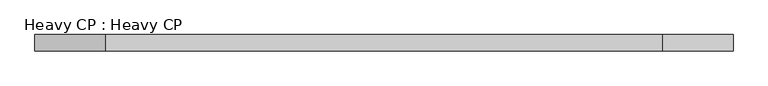
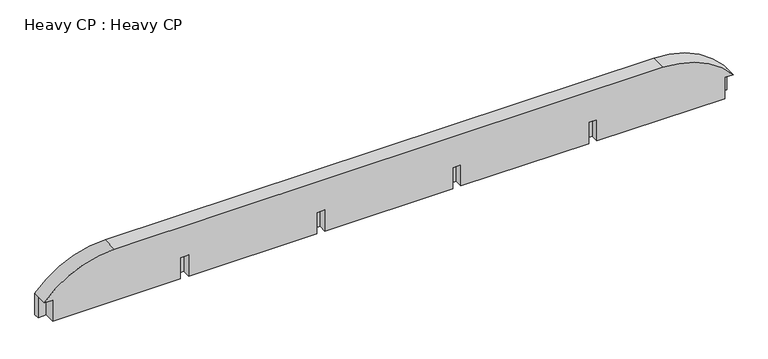
"""IFC4 building model written with IfcOpenShell, lengths in millimetres: beam geometry, Heavy CP : Heavy CP."""

from ifc_helpers import new_model, si_unit, frame, origin, place, context, project, spatial, circle_curve, source, transform, mapped, element, save
from ifc_brep_helpers import plane_surface, cylinder_surface, advanced_brep


def heavy_cp_heavy_cp_8a3f1562(model_context):
    return source(origin(), model_context, "Body", "AdvancedBrep", [
        advanced_brep(
        [(25183.2245516, 20299.9999993, 13800.0), (25183.2245516, 20299.9999993, 14620.0), (27758.2245515, 20299.9999993, 15800.827786), (47908.2245512, 20299.9999993, 15800.827786), (50483.2245514, 20299.9999993, 14619.9999997), (50483.2245514, 20299.9999993, 13800.0), (27583.2245516, 20299.9999993, 13800.0), (50483.2245514, 19699.9999993, 14619.9999997), (47908.2245512, 19699.9999993, 15800.827786), (27758.2245515, 19699.9999993, 15800.827786), (25183.2245516, 19699.9999993, 14620.0), (25483.2245516, 19699.9999993, 14620.0), (25483.2245516, 19699.9999993, 13800.0), (27583.2245516, 19699.9999993, 13800.0), (30183.2245515, 19699.9999993, 13800.0), (30183.2245515, 19699.9999993, 14620.0), (30333.2245515, 19699.9999993, 14620.0), (30483.2245515, 19699.9999993, 14620.0), (30483.2245515, 19699.9999993, 13800.0), (35183.2245514, 19699.9999993, 13800.0), (35183.2245514, 19699.9999993, 14620.0), (35483.2245514, 19699.9999993, 14620.0), (35483.2245514, 19699.9999993, 13800.0), (40183.2245513, 19699.9999993, 13800.0), (40183.2245513, 19699.9999993, 14620.0), (40483.2245513, 19699.9999993, 14620.0), (40483.2245513, 19699.9999993, 13800.0), (45183.2245512, 19699.9999993, 13800.0), (45183.2245512, 19699.9999993, 14620.0), (45483.2245512, 19699.9999993, 14620.0), (45483.2245512, 19699.9999993, 13800.0), (50183.2245511, 19699.9999993, 13800.0), (50183.2245511, 19699.9999993, 14620.0), (25183.2245516, 20099.7448193, 13800.0), (25183.2245516, 20099.7448193, 14620.0), (50483.2245511, 20099.7448193, 14620.0), (50483.2245514, 20099.7448193, 13800.0), (50183.2245511, 20099.7448193, 13800.0), (45483.2245512, 19999.9999993, 13800.0), (45183.2245512, 19999.9999993, 13800.0), (40483.2245513, 19999.9999993, 13800.0), (40183.2245513, 19999.9999993, 13800.0), (35483.2245514, 19999.9999993, 13800.0), (35183.2245514, 19999.9999993, 13800.0), (30483.2245515, 19999.9999993, 13800.0), (30183.2245515, 19999.9999993, 13800.0), (25483.2245516, 20099.7448193, 13800.0), (25483.2245516, 20099.7448193, 14620.0), (30483.2245515, 19999.9999993, 14620.0), (30183.2245515, 19999.9999993, 14620.0), (35483.2245514, 19999.9999993, 14620.0), (35183.2245514, 19999.9999993, 14620.0), (40483.2245513, 19999.9999993, 14620.0), (40183.2245513, 19999.9999993, 14620.0), (45483.2245512, 19999.9999993, 14620.0), (45183.2245512, 19999.9999993, 14620.0), (50183.2245511, 20099.7448193, 14620.0)],
        [
            (0, 1),
            (1, 2, circle_curve(frame((27758.2245515, 20299.9999993, 12402.7966103), z_axis=(0.0, 1.0, 0.0), x_axis=(0.0, 0.0, -1.0)), 3398.0311757)),
            (2, 3),
            (3, 4, circle_curve(frame((47908.2245512, 20299.9999993, 12402.7966102), z_axis=(0.0, 1.0, 0.0), x_axis=(0.0, 0.0, -1.0)), 3398.0311757)),
            (4, 5),
            (5, 6),
            (6, 0),
            (7, 8, circle_curve(frame((47908.2245512, 19699.9999993, 12402.7966102), z_axis=(0.0, -1.0, 0.0), x_axis=(0.0, 0.0, -1.0)), 3398.0311757)),
            (8, 9),
            (9, 10, circle_curve(frame((27758.2245515, 19699.9999993, 12402.7966103), z_axis=(0.0, -1.0, 0.0), x_axis=(0.0, 0.0, -1.0)), 3398.0311757)),
            (10, 11),
            (11, 12),
            (12, 13),
            (13, 14),
            (14, 15),
            (15, 16),
            (16, 17),
            (17, 18),
            (18, 19),
            (19, 20),
            (20, 21),
            (21, 22),
            (22, 23),
            (23, 24),
            (24, 25),
            (25, 26),
            (26, 27),
            (27, 28),
            (28, 29),
            (29, 30),
            (30, 31),
            (31, 32),
            (32, 7),
            (0, 33),
            (33, 34),
            (34, 1),
            (34, 10),
            (9, 2),
            (8, 3),
            (7, 35),
            (35, 4),
            (35, 36),
            (36, 5),
            (36, 37),
            (37, 31),
            (30, 38),
            (38, 39),
            (39, 27),
            (26, 40),
            (40, 41),
            (41, 23),
            (22, 42),
            (42, 43),
            (43, 19),
            (18, 44),
            (44, 45),
            (45, 14),
            (12, 46),
            (46, 33),
            (34, 47),
            (47, 11),
            (47, 46),
            (48, 49),
            (49, 45),
            (44, 48),
            (48, 17),
            (15, 49),
            (50, 51),
            (51, 43),
            (42, 50),
            (50, 21),
            (20, 51),
            (52, 53),
            (53, 41),
            (40, 52),
            (52, 25),
            (24, 53),
            (54, 55),
            (55, 39),
            (38, 54),
            (54, 29),
            (28, 55),
            (56, 35),
            (32, 56),
            (37, 56),
        ],
        [
            plane_surface(frame((25183.2245516, 20299.9999993, 13800.0), z_axis=(0.0, 1.0, 0.0), x_axis=(0.0, 0.0, 1.0))),
            plane_surface(frame((25183.2245516, 19699.9999993, 13800.0), z_axis=(0.0, -1.0, 0.0), x_axis=(0.0, 0.0, -1.0))),
            plane_surface(frame((25183.2245516, 20299.9999993, 13800.0), z_axis=(-1.0, 0.0, 0.0), x_axis=(0.0, -1.0, 0.0))),
            cylinder_surface(frame((27758.2245515, 19699.9999993, 12402.7966103), z_axis=(0.0, 1.0, 0.0), x_axis=(0.0, 0.0, -1.0)), 3398.0311757),
            plane_surface(frame((27758.2245515, 20299.9999993, 15800.827786), z_axis=(0.0, 0.0, 1.0), x_axis=(0.0, -1.0, 0.0))),
            cylinder_surface(frame((47908.2245512, 19699.9999993, 12402.7966102), z_axis=(0.0, 1.0, 0.0), x_axis=(0.0, 0.0, -1.0)), 3398.0311757),
            plane_surface(frame((50483.2245514, 20299.9999993, 14619.9999997), z_axis=(1.0, 0.0, 0.0), x_axis=(0.0, -1.0, 0.0))),
            plane_surface(frame((50483.2245514, 20299.9999993, 13800.0), z_axis=(0.0, 0.0, -1.0), x_axis=(0.0, -1.0, 0.0))),
            plane_surface(frame((25183.2245516, 19687.2999993, 14620.0), z_axis=(0.0, 0.0, -1.0), x_axis=(0.0, -1.0, 0.0))),
            plane_surface(frame((25483.2245516, 19687.2999993, 14620.0), z_axis=(-1.0, 0.0, 0.0), x_axis=(0.0, -1.0, 0.0))),
            plane_surface(frame((25333.2245516, 20099.7448193, 13800.0), z_axis=(0.0, -1.0, 0.0), x_axis=(0.0, 0.0, 1.0))),
            plane_surface(frame((30333.2245515, 19999.9999993, 14210.0), z_axis=(0.0, -1.0, 0.0), x_axis=(0.0, 0.0, 1.0))),
            plane_surface(frame((30183.2245515, 19999.9999993, 14620.0), z_axis=(0.0, 0.0, -1.0), x_axis=(0.0, -1.0, 0.0))),
            plane_surface(frame((30483.2245515, 19999.9999993, 14620.0), z_axis=(-1.0, 0.0, 0.0), x_axis=(0.0, -1.0, 0.0))),
            plane_surface(frame((30183.2245515, 19999.9999993, 13800.0), z_axis=(1.0, 0.0, 0.0), x_axis=(0.0, -1.0, 0.0))),
            plane_surface(frame((35333.2245514, 19999.9999993, 14210.0), z_axis=(0.0, -1.0, 0.0), x_axis=(0.0, 0.0, 1.0))),
            plane_surface(frame((35183.2245514, 19999.9999993, 14620.0), z_axis=(0.0, 0.0, -1.0), x_axis=(0.0, -1.0, 0.0))),
            plane_surface(frame((35483.2245514, 19999.9999993, 14620.0), z_axis=(-1.0, 0.0, 0.0), x_axis=(0.0, -1.0, 0.0))),
            plane_surface(frame((35183.2245514, 19999.9999993, 13800.0), z_axis=(1.0, 0.0, 0.0), x_axis=(0.0, -1.0, 0.0))),
            plane_surface(frame((40333.2245513, 19999.9999993, 14210.0), z_axis=(0.0, -1.0, 0.0), x_axis=(0.0, 0.0, 1.0))),
            plane_surface(frame((40183.2245513, 19999.9999993, 14620.0), z_axis=(0.0, 0.0, -1.0), x_axis=(0.0, -1.0, 0.0))),
            plane_surface(frame((40483.2245513, 19999.9999993, 14620.0), z_axis=(-1.0, 0.0, 0.0), x_axis=(0.0, -1.0, 0.0))),
            plane_surface(frame((40183.2245513, 19999.9999993, 13800.0), z_axis=(1.0, 0.0, 0.0), x_axis=(0.0, -1.0, 0.0))),
            plane_surface(frame((45333.2245512, 19999.9999993, 14210.0), z_axis=(0.0, -1.0, 0.0), x_axis=(0.0, 0.0, 1.0))),
            plane_surface(frame((45183.2245512, 19999.9999993, 14620.0), z_axis=(0.0, 0.0, -1.0), x_axis=(0.0, -1.0, 0.0))),
            plane_surface(frame((45483.2245512, 19999.9999993, 14620.0), z_axis=(-1.0, 0.0, 0.0), x_axis=(0.0, -1.0, 0.0))),
            plane_surface(frame((45183.2245512, 19999.9999993, 13800.0), z_axis=(1.0, 0.0, 0.0), x_axis=(0.0, -1.0, 0.0))),
            plane_surface(frame((50183.2245511, 19687.2999993, 14620.0), z_axis=(0.0, 0.0, -1.0), x_axis=(0.0, -1.0, 0.0))),
            plane_surface(frame((50183.2245511, 19687.2999993, 13800.0), z_axis=(1.0, 0.0, 0.0), x_axis=(0.0, -1.0, 0.0))),
            plane_surface(frame((50333.2245511, 20099.7448193, 13800.0), z_axis=(0.0, -1.0, 0.0), x_axis=(0.0, 0.0, 1.0))),
        ],
        [
            (0, [[1, 2, 3, 4, 5, 6, 7]]),
            (1, [[8, 9, 10, 11, 12, 13, 14, 15, 16, 17, 18, 19, 20, 21, 22, 23, 24, 25, 26, 27, 28, 29, 30, 31, 32, 33]]),
            (2, [[-1, 34, 35, 36]]),
            (3, [[-2, -36, 37, -10, 38]]),
            (4, [[-3, -38, -9, 39]]),
            (5, [[-4, -39, -8, 40, 41]]),
            (6, [[-5, -41, 42, 43]]),
            (7, [[-7, -6, -43, 44, 45, -31, 46, 47, 48, -27, 49, 50, 51, -23, 52, 53, 54, -19, 55, 56, 57, -14, -13, 58, 59, -34]]),
            (8, [[60, 61, -11, -37]]),
            (9, [[62, -58, -12, -61]]),
            (10, [[-60, -35, -59, -62]]),
            (11, [[63, 64, -56, 65]]),
            (12, [[-63, 66, -17, -16, 67]]),
            (13, [[-65, -55, -18, -66]]),
            (14, [[-64, -67, -15, -57]]),
            (15, [[68, 69, -53, 70]]),
            (16, [[-68, 71, -21, 72]]),
            (17, [[-70, -52, -22, -71]]),
            (18, [[-69, -72, -20, -54]]),
            (19, [[73, 74, -50, 75]]),
            (20, [[-73, 76, -25, 77]]),
            (21, [[-75, -49, -26, -76]]),
            (22, [[-74, -77, -24, -51]]),
            (23, [[78, 79, -47, 80]]),
            (24, [[-78, 81, -29, 82]]),
            (25, [[-80, -46, -30, -81]]),
            (26, [[-79, -82, -28, -48]]),
            (27, [[83, -40, -33, 84]]),
            (28, [[85, -84, -32, -45]]),
            (29, [[-83, -85, -44, -42]]),
        ],
    ),
    ])


if __name__ == "__main__":
    model = new_model("IFC4")
    model_context = context("Model", 3, world=origin())
    ifc_project = project(units=[si_unit("LENGTHUNIT", "METRE", prefix="MILLI")], contexts=[model_context])
    site = spatial("IfcSite", under=ifc_project)
    building = spatial("IfcBuilding", under=site)
    placement = place(None, origin())
    heavy_cp_heavy_cp_shape = heavy_cp_heavy_cp_8a3f1562(model_context)
    element("IfcBeam", 1, ObjectType="Heavy CP : Heavy CP", at=placement, inside=building, context=model_context, shape_type="MappedRepresentation", body=[
        mapped(heavy_cp_heavy_cp_shape, transform((0.0, 0.0, 0.0), x_axis=(1.0, 0.0, 0.0), y_axis=(0.0, 1.0, 0.0), z_axis=(0.0, 0.0, 1.0))),
    ])
    save(model, "model.ifc")
